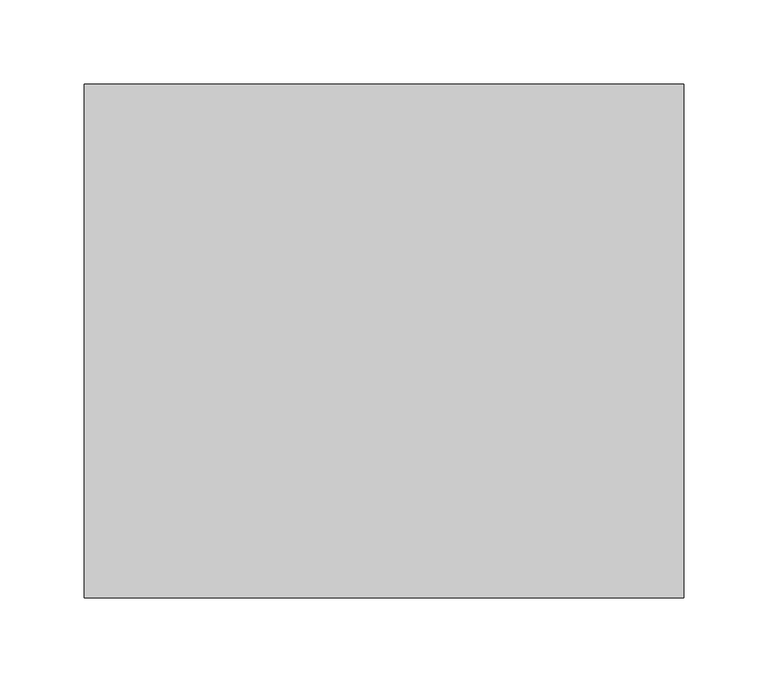
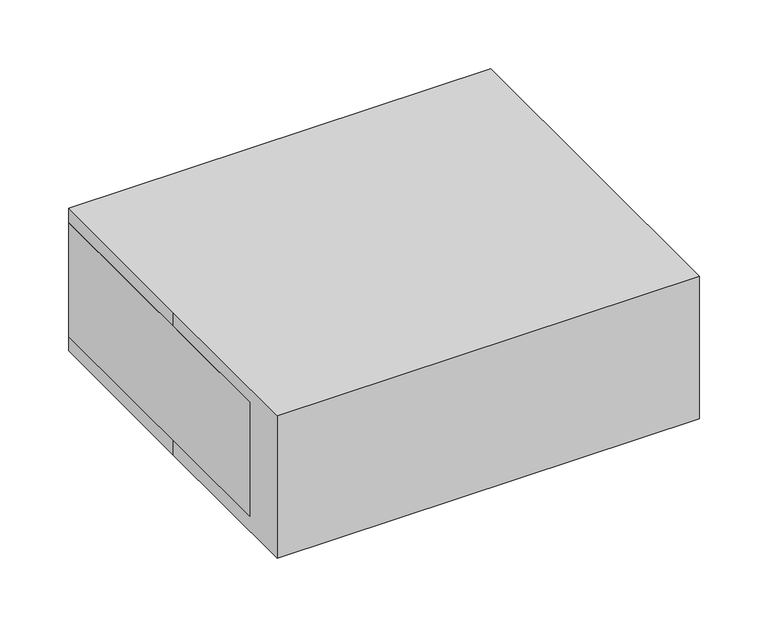
"""IFC4 building model written with IfcOpenShell, lengths in millimetres: proxy geometry, M8551 - Light Source, Fiberoptic Headlamp : M8551 - Light Source, Fiberoptic Headlamp."""

from ifc_helpers import new_model, si_unit, point, frame, frame_2d, origin, origin_with_axes, place, context, project, spatial, polyline, circle_curve, trimmed, segment, composite_curve, outline, extrude, source, transform, mapped, element, save


def specialty_equipment_4bd9d96e(model_context):
    return source(origin(), model_context, "Body", "SweptSolid", [
        extrude(outline(polyline([(142.2096017, -124.4389004), (97.7596017, -124.4389004), (97.7596017, -111.7389004), (142.2096017, -111.7389004), (142.2096017, -124.4389004)])), frame((0.0, 0.0, 40.6305658), z_axis=(0.0, 0.0, 1.0), x_axis=(1.0, 0.0, 0.0)), (0.0, 0.0, 1.0), 25.4),
        extrude(outline(polyline([(66.0096017, -124.4389004), (21.5596017, -124.4389004), (21.5596017, -111.7389004), (66.0096017, -111.7389004), (66.0096017, -124.4389004)])), frame((0.0, 0.0, 40.6305658), z_axis=(0.0, 0.0, 1.0), x_axis=(1.0, 0.0, 0.0)), (0.0, 0.0, 1.0), 25.4),
        extrude(outline(polyline([(122.6611094, -124.4389004), (52.8111094, -124.4389004), (52.8111094, -111.7389004), (122.6611094, -111.7389004), (122.6611094, -124.4389004)])), frame((0.0, 0.0, 87.4668281), z_axis=(0.0, 0.0, 1.0), x_axis=(1.0, 0.0, 0.0)), (0.0, 0.0, 1.0), 12.7),
        extrude(outline(composite_curve([segment(trimmed(circle_curve(frame_2d((69.3961128, -46.7129229)), 6.35), [point((69.3961128, -53.0629229))], [point((69.3961128, -40.3629229))], False, "CARTESIAN"), True, "CONTINUOUS"), segment(trimmed(circle_curve(frame_2d((69.3961128, -46.7129229)), 6.35), [point((69.3961128, -40.3629229))], [point((69.3961128, -53.0629229))], False, "CARTESIAN"), True, "CONTINUOUS")], self_intersect=False)), frame((0.0, -124.4389004, 0.0), z_axis=(0.0, 1.0, 0.0), x_axis=(0.0, 0.0, 1.0)), (0.0, 0.0, 1.0), 12.7),
        extrude(outline(composite_curve([segment(trimmed(circle_curve(frame_2d((67.9537355, -104.8888066)), 19.05), [point((67.9537355, -123.9388066))], [point((67.9537355, -85.8388066))], False, "CARTESIAN"), True, "CONTINUOUS"), segment(trimmed(circle_curve(frame_2d((67.9537355, -104.8888066)), 19.05), [point((67.9537355, -85.8388066))], [point((67.9537355, -123.9388066))], False, "CARTESIAN"), True, "CONTINUOUS")], self_intersect=False)), frame((0.0, -137.1389004, 0.0), z_axis=(0.0, 1.0, 0.0), x_axis=(0.0, 0.0, 1.0)), (0.0, 0.0, 1.0), 25.4),
        extrude(outline(composite_curve([segment(trimmed(circle_curve(frame_2d((137.9995251, -74.3090998)), 12.7), [point((150.6995251, -74.3090998))], [point((125.2995251, -74.3090998))], False, "CARTESIAN"), True, "CONTINUOUS"), segment(trimmed(circle_curve(frame_2d((137.9995251, -74.3090998)), 12.7), [point((125.2995251, -74.3090998))], [point((150.6995251, -74.3090998))], False, "CARTESIAN"), True, "CONTINUOUS")], self_intersect=False)), origin_with_axes(), (0.0, 0.0, 1.0), 12.7),
        extrude(outline(composite_curve([segment(trimmed(circle_curve(frame_2d((137.9995251, 116.1909002)), 12.7), [point((150.6995251, 116.1909002))], [point((125.2995251, 116.1909002))], False, "CARTESIAN"), True, "CONTINUOUS"), segment(trimmed(circle_curve(frame_2d((137.9995251, 116.1909002)), 12.7), [point((125.2995251, 116.1909002))], [point((150.6995251, 116.1909002))], False, "CARTESIAN"), True, "CONTINUOUS")], self_intersect=False)), origin_with_axes(), (0.0, 0.0, 1.0), 12.7),
        extrude(outline(composite_curve([segment(trimmed(circle_curve(frame_2d((-137.9995251, -74.3090998)), 12.7), [point((-150.6995251, -74.3090998))], [point((-125.2995251, -74.3090998))], False, "CARTESIAN"), True, "CONTINUOUS"), segment(trimmed(circle_curve(frame_2d((-137.9995251, -74.3090998)), 12.7), [point((-125.2995251, -74.3090998))], [point((-150.6995251, -74.3090998))], False, "CARTESIAN"), True, "CONTINUOUS")], self_intersect=False)), origin_with_axes(), (0.0, 0.0, 1.0), 12.7),
        extrude(outline(polyline([(177.8, 152.4), (177.8, -111.7389004), (-177.8, -111.7389004), (-177.8, 152.4), (177.8, 152.4)])), frame((0.0, 0.0, 12.7), z_axis=(0.0, 0.0, 1.0), x_axis=(1.0, 0.0, 0.0)), (0.0, 0.0, 1.0), 101.6),
        extrude(outline(composite_curve([segment(trimmed(circle_curve(frame_2d((-137.9995251, 116.1909002)), 12.7), [point((-150.6995251, 116.1909002))], [point((-125.2995251, 116.1909002))], False, "CARTESIAN"), True, "CONTINUOUS"), segment(trimmed(circle_curve(frame_2d((-137.9995251, 116.1909002)), 12.7), [point((-125.2995251, 116.1909002))], [point((-150.6995251, 116.1909002))], False, "CARTESIAN"), True, "CONTINUOUS")], self_intersect=False)), origin_with_axes(), (0.0, 0.0, 1.0), 12.7),
        extrude(outline(polyline([(-177.8, 152.4), (177.8, 152.4), (177.8, -152.4), (-177.8, -152.4), (-177.8, 0.0), (-177.8, 152.4)])), origin_with_axes(), (0.0, 0.0, 1.0), 127.0),
    ])


if __name__ == "__main__":
    model = new_model("IFC4")
    model_context = context("Model", 3, world=origin())
    ifc_project = project(units=[si_unit("LENGTHUNIT", "METRE", prefix="MILLI")], contexts=[model_context])
    site = spatial("IfcSite", under=ifc_project)
    building = spatial("IfcBuilding", under=site)
    placement = place(None, origin())
    specialty_equipment_shape = specialty_equipment_4bd9d96e(model_context)
    element("IfcBuildingElementProxy", 1, Name="M8551 - Light Source, Fiberoptic Headlamp : M8551 - Light Source, Fiberoptic Headlamp", ObjectType="M8551 - Light Source, Fiberoptic Headlamp : M8551 - Light Source, Fiberoptic Headlamp", at=placement, inside=building, context=model_context, shape_type="MappedRepresentation", body=[
        mapped(specialty_equipment_shape, transform((0.0, 0.0, 0.0), x_axis=(1.0, 0.0, 0.0), y_axis=(0.0, 1.0, 0.0), z_axis=(0.0, 0.0, 1.0))),
    ])
    save(model, "model.ifc")

# Revit data of these elements
# Type "M8551 - Light Source, Fiberoptic Headlamp : M8551 - Light Source, Fiberoptic Headlamp"
#   Watts2 = "0"
#   Watts1 = "720"
#   Unit_Issue = "EA"
#   UTIL_6_Misc = "-"
#   UTIL_5_NonMedGas = "-"
#   UTIL_4_MiscGas = "-"
#   UTIL_3_MedGas = "-"
#   UTIL_2_Elec = "A"
#   UTIL_1_WaterDrain = "-"
#   Nomenclature = "Light Source, Fiberoptic Headlamp"
#   NSN = "6515"
#   Location [instance default] = ""
#   JSN = "M8551"
#   Fund_Source_VA = "-"
#   Fund_Source_Navy = "-"
#   Fund_Source_Army = "-"
#   Fund_Source_AF = "-"
#   ELEC_Volts2 = "0"
#   ELEC_Volts1 = "120"
#   ELEC_Phase2 = "0"
#   ELEC_Phase1 = "1"
#   ELEC_HertzSwitch = "-1"
#   ELEC_HertzDependent = "-1"
#   ELEC_Hertz = "60"
#   ELEC_Amps2 = "0"
#   ELEC_Amps1 = "6"
#   DetailDescription = "Fiberoptic light source for surgical headlamps. This unit provides color corrected light for surgical procedures where photography is not required."
#   CAT_VA = "C"
#   CAT_Navy = "C"
#   CAT_IHS = "-"
#   CAT_Army = "C"
#   CAT_AF = "C"
#   BTUperhour = "0"
#   Weight_IP = 14
#   DIM_Width_IP = 1' - 2"
#   DIM_Height_IP = 0' - 5"
#   DIM_Depth_IP = 1' - 0"
#   finish [instance default] = none
# Element 1 (IfcBuildingElementProxy, "M8551 - Light Source, Fiberoptic Headlamp : M8551 - Light Source, Fiberoptic Headlamp")
#   Location = "ORCS1"
#   Materials on its faces: "EquipSpace"
# Materials
#   "EquipSpace": class "Unassigned", colour RGB 221 217 195, transparency 0.5
